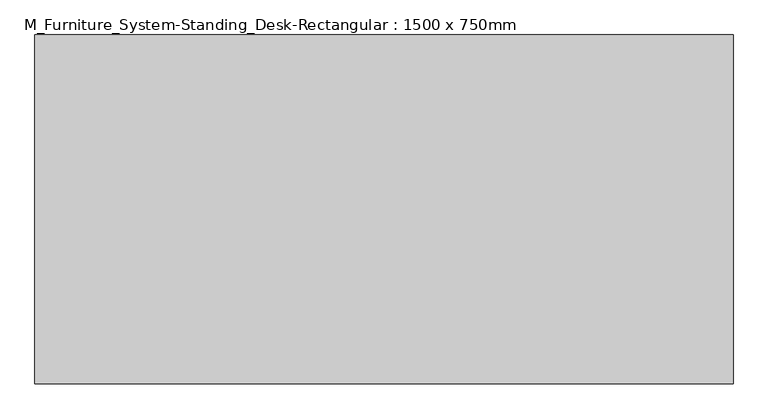
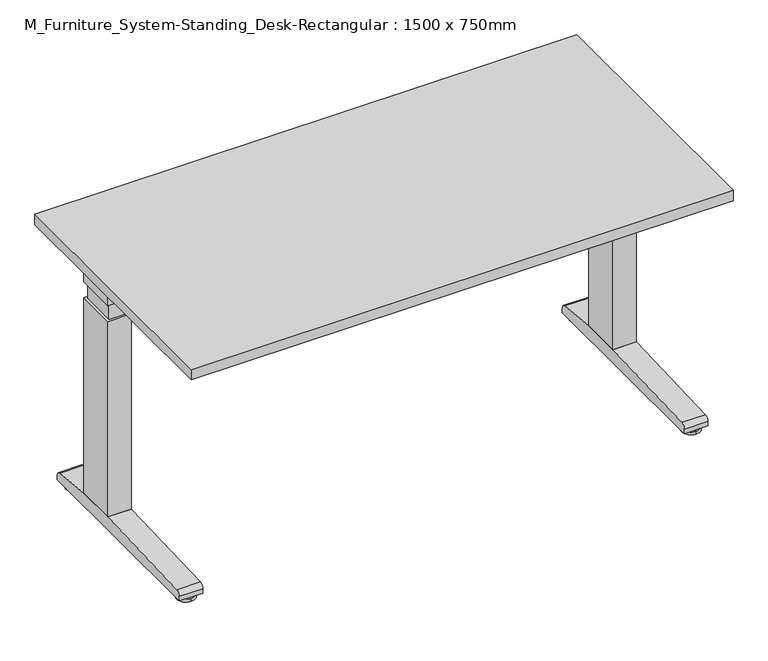
"""IFC4 building model written with IfcOpenShell, lengths in millimetres: furniture geometry, M_Furniture_System-Standing_Desk-Rectangular : 1500 x 750mm."""

from ifc_helpers import new_model, si_unit, point, frame, frame_2d, origin, place, context, project, spatial, polyline, circle_curve, trimmed, segment, composite_curve, outline, extrude, source, transform, mapped, element, save
from ifc_brep_helpers import plane_surface, cylinder_surface, advanced_brep


def m_furniture_system_standing_desk_rectangular_1500_x_750mm_4d5fce88(model_context):
    return source(origin(), model_context, "Body", "SolidModel", [
        advanced_brep(
        [(50.8, -610.3, 0.0), (50.8, -661.1, 0.0), (50.8, -635.7, 0.0), (50.8, -610.3, 8.4666667), (50.8, -661.1, 8.4666667), (50.8, -631.4666667, 8.4666667), (50.8, -639.9333333, 8.4666667), (50.8, -631.4666667, 12.7), (50.8, -639.9333333, 12.7), (50.8, -635.7, 12.7)],
        [
            (0, 1, circle_curve(frame((50.8, -635.7, 0.0), z_axis=(0.0, 0.0, -1.0), x_axis=(0.0, -1.0000000000000004, 0.0)), 25.4)),
            (1, 2),
            (2, 0),
            (1, 0, circle_curve(frame((50.8, -635.7, 0.0), z_axis=(0.0, 0.0, -1.0), x_axis=(0.0, -1.0000000000000004, 0.0)), 25.4)),
            (3, 4, circle_curve(frame((50.8, -635.7, 8.4666667), z_axis=(0.0, 0.0, -1.0), x_axis=(0.0, -1.0000000000000004, 0.0)), 25.4)),
            (4, 1),
            (0, 3),
            (4, 3, circle_curve(frame((50.8, -635.7, 8.4666667), z_axis=(0.0, 0.0, -1.0), x_axis=(0.0, -1.0000000000000004, 0.0)), 25.4)),
            (5, 6, circle_curve(frame((50.8, -635.7, 8.4666667), z_axis=(0.0, 0.0, -1.0), x_axis=(0.0, -1.0000000000000004, 0.0)), 4.2333333)),
            (6, 4),
            (3, 5),
            (6, 5, circle_curve(frame((50.8, -635.7, 8.4666667), z_axis=(0.0, 0.0, -1.0), x_axis=(0.0, -1.0000000000000004, 0.0)), 4.2333333)),
            (7, 8, circle_curve(frame((50.8, -635.7, 12.7), z_axis=(0.0, 0.0, -1.0), x_axis=(0.0, -1.0000000000000004, 0.0)), 4.2333333)),
            (8, 6),
            (5, 7),
            (8, 7, circle_curve(frame((50.8, -635.7, 12.7), z_axis=(0.0, 0.0, -1.0), x_axis=(0.0, -1.0000000000000004, 0.0)), 4.2333333)),
            (9, 8),
            (7, 9),
        ],
        [
            plane_surface(frame((50.8, -635.7, 0.0), z_axis=(0.0, 0.0, -1.0), x_axis=(0.0, -1.0, 0.0))),
            cylinder_surface(frame((50.8, -635.7, 69.85), z_axis=(0.0, 0.0, 1.0), x_axis=(0.0, -1.0000000000000004, 0.0)), 25.4),
            plane_surface(frame((50.8, -635.7, 8.4666667), z_axis=(0.0, 0.0, 1.0), x_axis=(0.0, -1.0, 0.0))),
            cylinder_surface(frame((50.8, -635.7, 69.85), z_axis=(0.0, 0.0, 1.0), x_axis=(0.0, -1.0000000000000004, 0.0)), 4.2333333),
            plane_surface(frame((50.8, -635.7, 12.7), z_axis=(0.0, 0.0, 1.0), x_axis=(0.0, -1.0, 0.0))),
        ],
        [
            (0, [[1, 2, 3]]),
            (0, [[4, -3, -2]]),
            (1, [[5, 6, -1, 7]]),
            (1, [[8, -7, -4, -6]]),
            (2, [[9, 10, -5, 11]]),
            (2, [[12, -11, -8, -10]]),
            (3, [[13, 14, -9, 15]]),
            (3, [[16, -15, -12, -14]]),
            (4, [[17, -13, 18]]),
            (4, [[-18, -16, -17]]),
        ],
    ),
        advanced_brep(
        [(50.8, -127.0, 0.0), (50.8, -76.2, 0.0), (50.8, -76.2, 8.4666667), (50.8, -127.0, 8.4666667), (50.8, -97.3666667, 8.4666667), (50.8, -105.8333333, 8.4666667), (50.8, -97.3666667, 12.7), (50.8, -105.8333333, 12.7), (50.8, -101.6, 12.7), (50.8, -101.6, 0.0)],
        [
            (0, 1, circle_curve(frame((50.8, -101.6, 0.0), z_axis=(0.0, 0.0, 1.0), x_axis=(0.0, 1.0000000000000004, 0.0)), 25.4)),
            (1, 2),
            (2, 3, circle_curve(frame((50.8, -101.6, 8.4666667), z_axis=(0.0, 0.0, -1.0), x_axis=(0.0, 1.0000000000000004, 0.0)), 25.4)),
            (3, 0),
            (1, 0, circle_curve(frame((50.8, -101.6, 0.0), z_axis=(0.0, 0.0, 1.0), x_axis=(0.0, 1.0000000000000004, 0.0)), 25.4)),
            (3, 2, circle_curve(frame((50.8, -101.6, 8.4666667), z_axis=(0.0, 0.0, -1.0), x_axis=(0.0, 1.0000000000000004, 0.0)), 25.4)),
            (2, 4),
            (4, 5, circle_curve(frame((50.8, -101.6, 8.4666667), z_axis=(0.0, 0.0, -1.0), x_axis=(0.0, 1.0000000000000004, 0.0)), 4.2333333)),
            (5, 3),
            (5, 4, circle_curve(frame((50.8, -101.6, 8.4666667), z_axis=(0.0, 0.0, -1.0), x_axis=(0.0, 1.0000000000000004, 0.0)), 4.2333333)),
            (4, 6),
            (6, 7, circle_curve(frame((50.8, -101.6, 12.7), z_axis=(0.0, 0.0, -1.0), x_axis=(0.0, 1.0000000000000004, 0.0)), 4.2333333)),
            (7, 5),
            (7, 6, circle_curve(frame((50.8, -101.6, 12.7), z_axis=(0.0, 0.0, -1.0), x_axis=(0.0, 1.0000000000000004, 0.0)), 4.2333333)),
            (6, 8),
            (8, 7),
            (9, 1),
            (0, 9),
        ],
        [
            cylinder_surface(frame((50.8, -101.6, 114.3), z_axis=(0.0, 0.0, -1.0), x_axis=(0.0, 1.0000000000000004, 0.0)), 25.4),
            plane_surface(frame((50.8, -101.6, 8.4666667), z_axis=(0.0, 0.0, 1.0), x_axis=(0.0, 1.0, 0.0))),
            cylinder_surface(frame((50.8, -101.6, 114.3), z_axis=(0.0, 0.0, -1.0), x_axis=(0.0, 1.0000000000000004, 0.0)), 4.2333333),
            plane_surface(frame((50.8, -101.6, 12.7), z_axis=(0.0, 0.0, 1.0), x_axis=(0.0, 1.0, 0.0))),
            plane_surface(frame((50.8, -101.6, 0.0), z_axis=(0.0, 0.0, -1.0), x_axis=(0.0, 1.0, 0.0))),
        ],
        [
            (0, [[1, 2, 3, 4]]),
            (0, [[5, -4, 6, -2]]),
            (1, [[-3, 7, 8, 9]]),
            (1, [[-6, -9, 10, -7]]),
            (2, [[-8, 11, 12, 13]]),
            (2, [[-10, -13, 14, -11]]),
            (3, [[-12, 15, 16]]),
            (3, [[-14, -16, -15]]),
            (4, [[17, -1, 18]]),
            (4, [[-18, -5, -17]]),
        ],
    ),
        extrude(outline(polyline([(83.3, -318.2), (18.3, -318.2), (18.3, -203.2), (83.3, -203.2), (83.3, -318.2)])), frame((0.0, 0.0, 669.2), z_axis=(0.0, 0.0, 1.0), x_axis=(1.0, 0.0, 0.0)), (0.0, 0.0, 1.0), 50.8),
        extrude(outline(polyline([(76.95, -311.85), (24.65, -311.85), (24.65, -209.55), (76.95, -209.55), (76.95, -311.85)])), frame((0.0, 0.0, 622.3), z_axis=(0.0, 0.0, 1.0), x_axis=(1.0, 0.0, 0.0)), (0.0, 0.0, 1.0), 46.9),
        extrude(outline(composite_curve([segment(polyline([(-661.1, 12.7), (-661.1, 25.8616628)]), True, "CONTINUOUS"), segment(trimmed(circle_curve(frame_2d((-648.4, 25.8616628)), 12.7), [point((-661.1, 25.8616628))], [point((-648.8700481, 38.5529612))], False, "CARTESIAN"), True, "CONTINUOUS"), segment(polyline([(-648.8700481, 38.5529612), (-318.2, 50.8), (-203.2, 50.8), (-87.6363028, 39.2436303)]), True, "CONTINUOUS"), segment(trimmed(circle_curve(frame_2d((-88.9, 26.606658)), 12.7), [point((-87.6363028, 39.2436303))], [point((-76.2, 26.606658))], False, "CARTESIAN"), True, "CONTINUOUS"), segment(polyline([(-76.2, 26.606658), (-76.2, 12.7), (-661.1, 12.7)]), True, "CONTINUOUS")], self_intersect=False)), frame((18.3, 0.0, 0.0), z_axis=(1.0, 0.0, 0.0), x_axis=(0.0, 1.0, 0.0)), (0.0, 0.0, 1.0), 65.0),
        extrude(outline(polyline([(83.3, -318.2), (18.3, -318.2), (18.3, -203.2), (83.3, -203.2), (83.3, -318.2)])), frame((0.0, 0.0, 50.8), z_axis=(0.0, 0.0, 1.0), x_axis=(1.0, 0.0, 0.0)), (0.0, 0.0, 1.0), 571.5),
        advanced_brep(
        [(1449.2, -610.3, 0.0), (1449.2, -661.1, 0.0), (1449.2, -635.7, 0.0), (1449.2, -610.3, 8.4666667), (1449.2, -661.1, 8.4666667), (1449.2, -631.4666667, 8.4666667), (1449.2, -639.9333333, 8.4666667), (1449.2, -631.4666667, 12.7), (1449.2, -639.9333333, 12.7), (1449.2, -635.7, 12.7)],
        [
            (0, 1, circle_curve(frame((1449.2, -635.7, 0.0), z_axis=(0.0, 0.0, -1.0), x_axis=(0.0, -1.0000000000000004, 0.0)), 25.4)),
            (1, 2),
            (2, 0),
            (1, 0, circle_curve(frame((1449.2, -635.7, 0.0), z_axis=(0.0, 0.0, -1.0), x_axis=(0.0, -1.0000000000000004, 0.0)), 25.4)),
            (3, 4, circle_curve(frame((1449.2, -635.7, 8.4666667), z_axis=(0.0, 0.0, -1.0), x_axis=(0.0, -1.0000000000000004, 0.0)), 25.4)),
            (4, 1),
            (0, 3),
            (4, 3, circle_curve(frame((1449.2, -635.7, 8.4666667), z_axis=(0.0, 0.0, -1.0), x_axis=(0.0, -1.0000000000000004, 0.0)), 25.4)),
            (5, 6, circle_curve(frame((1449.2, -635.7, 8.4666667), z_axis=(0.0, 0.0, -1.0), x_axis=(0.0, -1.0000000000000004, 0.0)), 4.2333333)),
            (6, 4),
            (3, 5),
            (6, 5, circle_curve(frame((1449.2, -635.7, 8.4666667), z_axis=(0.0, 0.0, -1.0), x_axis=(0.0, -1.0000000000000004, 0.0)), 4.2333333)),
            (7, 8, circle_curve(frame((1449.2, -635.7, 12.7), z_axis=(0.0, 0.0, -1.0), x_axis=(0.0, -1.0000000000000004, 0.0)), 4.2333333)),
            (8, 6),
            (5, 7),
            (8, 7, circle_curve(frame((1449.2, -635.7, 12.7), z_axis=(0.0, 0.0, -1.0), x_axis=(0.0, -1.0000000000000004, 0.0)), 4.2333333)),
            (9, 8),
            (7, 9),
        ],
        [
            plane_surface(frame((1449.2, -635.7, 0.0), z_axis=(0.0, 0.0, -1.0), x_axis=(0.0, -1.0, 0.0))),
            cylinder_surface(frame((1449.2, -635.7, 69.85), z_axis=(0.0, 0.0, 1.0), x_axis=(0.0, -1.0000000000000004, 0.0)), 25.4),
            plane_surface(frame((1449.2, -635.7, 8.4666667), z_axis=(0.0, 0.0, 1.0), x_axis=(0.0, -1.0, 0.0))),
            cylinder_surface(frame((1449.2, -635.7, 69.85), z_axis=(0.0, 0.0, 1.0), x_axis=(0.0, -1.0000000000000004, 0.0)), 4.2333333),
            plane_surface(frame((1449.2, -635.7, 12.7), z_axis=(0.0, 0.0, 1.0), x_axis=(0.0, -1.0, 0.0))),
        ],
        [
            (0, [[1, 2, 3]]),
            (0, [[4, -3, -2]]),
            (1, [[5, 6, -1, 7]]),
            (1, [[8, -7, -4, -6]]),
            (2, [[9, 10, -5, 11]]),
            (2, [[12, -11, -8, -10]]),
            (3, [[13, 14, -9, 15]]),
            (3, [[16, -15, -12, -14]]),
            (4, [[17, -13, 18]]),
            (4, [[-18, -16, -17]]),
        ],
    ),
        advanced_brep(
        [(1449.2, -127.0, 0.0), (1449.2, -76.2, 0.0), (1449.2, -76.2, 8.4666667), (1449.2, -127.0, 8.4666667), (1449.2, -97.3666667, 8.4666667), (1449.2, -105.8333333, 8.4666667), (1449.2, -97.3666667, 12.7), (1449.2, -105.8333333, 12.7), (1449.2, -101.6, 12.7), (1449.2, -101.6, 0.0)],
        [
            (0, 1, circle_curve(frame((1449.2, -101.6, 0.0), z_axis=(0.0, 0.0, 1.0), x_axis=(0.0, 1.0000000000000004, 0.0)), 25.4)),
            (1, 2),
            (2, 3, circle_curve(frame((1449.2, -101.6, 8.4666667), z_axis=(0.0, 0.0, -1.0), x_axis=(0.0, 1.0000000000000004, 0.0)), 25.4)),
            (3, 0),
            (1, 0, circle_curve(frame((1449.2, -101.6, 0.0), z_axis=(0.0, 0.0, 1.0), x_axis=(0.0, 1.0000000000000004, 0.0)), 25.4)),
            (3, 2, circle_curve(frame((1449.2, -101.6, 8.4666667), z_axis=(0.0, 0.0, -1.0), x_axis=(0.0, 1.0000000000000004, 0.0)), 25.4)),
            (2, 4),
            (4, 5, circle_curve(frame((1449.2, -101.6, 8.4666667), z_axis=(0.0, 0.0, -1.0), x_axis=(0.0, 1.0000000000000004, 0.0)), 4.2333333)),
            (5, 3),
            (5, 4, circle_curve(frame((1449.2, -101.6, 8.4666667), z_axis=(0.0, 0.0, -1.0), x_axis=(0.0, 1.0000000000000004, 0.0)), 4.2333333)),
            (4, 6),
            (6, 7, circle_curve(frame((1449.2, -101.6, 12.7), z_axis=(0.0, 0.0, -1.0), x_axis=(0.0, 1.0000000000000004, 0.0)), 4.2333333)),
            (7, 5),
            (7, 6, circle_curve(frame((1449.2, -101.6, 12.7), z_axis=(0.0, 0.0, -1.0), x_axis=(0.0, 1.0000000000000004, 0.0)), 4.2333333)),
            (6, 8),
            (8, 7),
            (9, 1),
            (0, 9),
        ],
        [
            cylinder_surface(frame((1449.2, -101.6, 114.3), z_axis=(0.0, 0.0, -1.0), x_axis=(0.0, 1.0000000000000004, 0.0)), 25.4),
            plane_surface(frame((1449.2, -101.6, 8.4666667), z_axis=(0.0, 0.0, 1.0), x_axis=(0.0, 1.0, 0.0))),
            cylinder_surface(frame((1449.2, -101.6, 114.3), z_axis=(0.0, 0.0, -1.0), x_axis=(0.0, 1.0000000000000004, 0.0)), 4.2333333),
            plane_surface(frame((1449.2, -101.6, 12.7), z_axis=(0.0, 0.0, 1.0), x_axis=(0.0, 1.0, 0.0))),
            plane_surface(frame((1449.2, -101.6, 0.0), z_axis=(0.0, 0.0, -1.0), x_axis=(0.0, 1.0, 0.0))),
        ],
        [
            (0, [[1, 2, 3, 4]]),
            (0, [[5, -4, 6, -2]]),
            (1, [[-3, 7, 8, 9]]),
            (1, [[-6, -9, 10, -7]]),
            (2, [[-8, 11, 12, 13]]),
            (2, [[-10, -13, 14, -11]]),
            (3, [[-12, 15, 16]]),
            (3, [[-14, -16, -15]]),
            (4, [[17, -1, 18]]),
            (4, [[-18, -5, -17]]),
        ],
    ),
        extrude(outline(polyline([(1481.7, -318.2), (1416.7, -318.2), (1416.7, -203.2), (1481.7, -203.2), (1481.7, -318.2)])), frame((0.0, 0.0, 669.2), z_axis=(0.0, 0.0, 1.0), x_axis=(1.0, 0.0, 0.0)), (0.0, 0.0, 1.0), 50.8),
        extrude(outline(polyline([(1475.35, -311.85), (1423.05, -311.85), (1423.05, -209.55), (1475.35, -209.55), (1475.35, -311.85)])), frame((0.0, 0.0, 622.3), z_axis=(0.0, 0.0, 1.0), x_axis=(1.0, 0.0, 0.0)), (0.0, 0.0, 1.0), 46.9),
        extrude(outline(composite_curve([segment(polyline([(-661.1, 12.7), (-661.1, 25.8616628)]), True, "CONTINUOUS"), segment(trimmed(circle_curve(frame_2d((-648.4, 25.8616628)), 12.7), [point((-661.1, 25.8616628))], [point((-648.8700481, 38.5529612))], False, "CARTESIAN"), True, "CONTINUOUS"), segment(polyline([(-648.8700481, 38.5529612), (-318.2, 50.8), (-203.2, 50.8), (-87.6363028, 39.2436303)]), True, "CONTINUOUS"), segment(trimmed(circle_curve(frame_2d((-88.9, 26.606658)), 12.7), [point((-87.6363028, 39.2436303))], [point((-76.2, 26.606658))], False, "CARTESIAN"), True, "CONTINUOUS"), segment(polyline([(-76.2, 26.606658), (-76.2, 12.7), (-661.1, 12.7)]), True, "CONTINUOUS")], self_intersect=False)), frame((1416.7, 0.0, 0.0), z_axis=(1.0, 0.0, 0.0), x_axis=(0.0, 1.0, 0.0)), (0.0, 0.0, 1.0), 65.0),
        extrude(outline(polyline([(1481.7, -318.2), (1416.7, -318.2), (1416.7, -203.2), (1481.7, -203.2), (1481.7, -318.2)])), frame((0.0, 0.0, 50.8), z_axis=(0.0, 0.0, 1.0), x_axis=(1.0, 0.0, 0.0)), (0.0, 0.0, 1.0), 571.5),
        extrude(outline(polyline([(1500.0, 0.0), (1500.0, -750.0), (0.0, -750.0), (0.0, 0.0), (1500.0, 0.0)])), frame((0.0, 0.0, 720.0), z_axis=(0.0, 0.0, 1.0), x_axis=(1.0, 0.0, 0.0)), (0.0, 0.0, 1.0), 30.0),
    ])


if __name__ == "__main__":
    model = new_model("IFC4")
    model_context = context("Model", 3, world=origin())
    ifc_project = project(units=[si_unit("LENGTHUNIT", "METRE", prefix="MILLI")], contexts=[model_context])
    site = spatial("IfcSite", under=ifc_project)
    building = spatial("IfcBuilding", under=site)
    placement = place(None, origin())
    m_furniture_system_standing_desk_rectangular_1500_x_750mm_shape = m_furniture_system_standing_desk_rectangular_1500_x_750mm_4d5fce88(model_context)
    element("IfcFurniture", 1, ObjectType="M_Furniture_System-Standing_Desk-Rectangular : 1500 x 750mm", at=placement, inside=building, context=model_context, shape_type="MappedRepresentation", body=[
        mapped(m_furniture_system_standing_desk_rectangular_1500_x_750mm_shape, transform((0.0, 0.0, 0.0), x_axis=(1.0, 0.0, 0.0), y_axis=(0.0, 1.0, 0.0), z_axis=(0.0, 0.0, 1.0))),
    ])
    save(model, "model.ifc")

# Revit data of these elements
# Type "M_Furniture_System-Standing_Desk-Rectangular : 1500 x 750mm"
#   Type Comments = "1500 x 750mm Rectangular Standing Desk"
#   Thickness = 30 mm
#   Width = 1500 mm
#   Height [instance default] = 750 mm
#   H [instance default] = 755 mm
#   Foot Height [instance default] = 720 mm
#   Depth = 750 mm
#   Work Surface Material [instance default] = Plastic Laminate - White Oak
#   Foot Material [instance default] = Metal - Paint Linen
#   Edge Material [instance default] = Plastic Laminate - Beige - Light - Smooth
#   Model = ""
#   Manufacturer = ""
#   Description = (empty or 0)
#   Default Elevation = 0
# Element 1 (IfcFurniture, "M_Furniture_System-Standing_Desk-Rectangular : 1500 x 750mm")
#   Work Surface Material = Ping Pong Table - Supports
#   Materials on its faces: "Metal - Paint Linen", "Plastic Laminate - Beige - Light - Smooth", "Ping Pong Table - Supports"
# Materials
#   "Plastic Laminate - White Oak": class "Wood", colour RGB 197 170 136, transparency 0
#   "Metal - Paint Linen": class "Metal", colour RGB 244 234 229, transparency 0
#   "Plastic Laminate - Beige - Light - Smooth": class "Plastic", colour RGB 215 199 171, transparency 0
#   "Ping Pong Table - Supports": class "Miscellaneous", colour RGB 255 255 255, transparency 0
